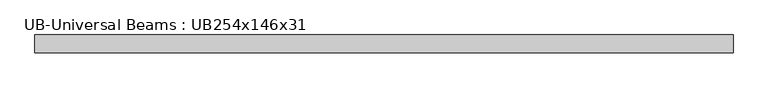
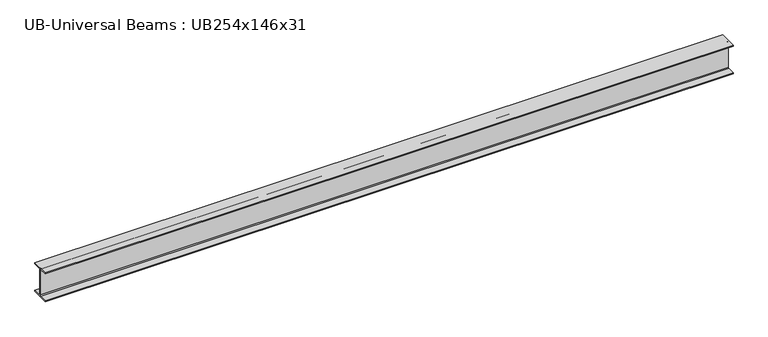
"""IFC4 building model written with IfcOpenShell, lengths in millimetres: beam geometry, UB-Universal Beams : UB254x146x31."""

from ifc_helpers import new_model, si_unit, point, frame, frame_2d, origin, place, context, project, spatial, polyline, circle_curve, trimmed, segment, composite_curve, outline, extrude, source, transform, mapped, element, save


def ub_universal_beams_ub254x146x31_048477c2(model_context):
    return source(origin(), model_context, "Body", "SweptSolid", [
        extrude(outline(composite_curve([segment(polyline([(73.05, -117.1), (73.05, -125.7), (-73.05, -125.7), (-73.05, -117.1), (-10.6, -117.1)]), True, "CONTINUOUS"), segment(trimmed(circle_curve(frame_2d((-10.6, -109.5)), 7.6), [point((-10.6, -117.1))], [point((-3.0, -109.5))], True, "CARTESIAN"), True, "CONTINUOUS"), segment(polyline([(-3.0, -109.5), (-3.0, 109.5)]), True, "CONTINUOUS"), segment(trimmed(circle_curve(frame_2d((-10.6, 109.5)), 7.6), [point((-3.0, 109.5))], [point((-10.6, 117.1))], True, "CARTESIAN"), True, "CONTINUOUS"), segment(polyline([(-10.6, 117.1), (-73.05, 117.1), (-73.05, 125.7), (73.05, 125.7), (73.05, 117.1), (10.6, 117.1)]), True, "CONTINUOUS"), segment(trimmed(circle_curve(frame_2d((10.6, 109.5)), 7.6), [point((10.6, 117.1))], [point((3.0, 109.5))], True, "CARTESIAN"), True, "CONTINUOUS"), segment(polyline([(3.0, 109.5), (3.0, -109.5)]), True, "CONTINUOUS"), segment(trimmed(circle_curve(frame_2d((10.6, -109.5)), 7.6), [point((3.0, -109.5))], [point((10.6, -117.1))], True, "CARTESIAN"), True, "CONTINUOUS"), segment(polyline([(10.6, -117.1), (73.05, -117.1)]), True, "CONTINUOUS")], self_intersect=False)), frame((-2847.0, 0.0, 0.0), z_axis=(1.0, 0.0, 0.0), x_axis=(0.0, 1.0, 0.0)), (0.0, 0.0, 1.0), 5694.0),
    ])


if __name__ == "__main__":
    model = new_model("IFC4")
    model_context = context("Model", 3, world=origin())
    ifc_project = project(units=[si_unit("LENGTHUNIT", "METRE", prefix="MILLI")], contexts=[model_context])
    site = spatial("IfcSite", under=ifc_project)
    building = spatial("IfcBuilding", under=site)
    placement = place(None, origin())
    ub_universal_beams_ub254x146x31_shape = ub_universal_beams_ub254x146x31_048477c2(model_context)
    element("IfcBeam", 1, ObjectType="UB-Universal Beams : UB254x146x31", at=placement, inside=building, context=model_context, shape_type="MappedRepresentation", body=[
        mapped(ub_universal_beams_ub254x146x31_shape, transform((0.0, 0.0, 0.0), x_axis=(1.0, 0.0, 0.0), y_axis=(0.0, 1.0, 0.0), z_axis=(0.0, 0.0, 1.0))),
    ])
    save(model, "model.ifc")

# Revit data of these elements
# Type "UB-Universal Beams : UB254x146x31"
#   Section Name Key = "UB254X146X31"
#   Width = 14.61 cm
#   Web Thickness = 0.6 cm
#   Web Fillet = 0.76 cm
#   Warping Constant = 66000.0 cm⁶
#   Torsional Moment of Inertia = 8.55 cm⁴
#   Section Area = 39.7 cm²
#   Plastic Modulus weak axis = 94.1 cm³
#   Plastic Modulus strong axis = 393.0 cm³
#   Nominal Weight = 31.10 kgf/m
#   Moment of Inertia weak axis = 448.00 cm⁴
#   Moment of Inertia strong axis = 4413.00 cm⁴
#   Height = 25.14 cm
#   Flange Thickness = 0.86 cm
#   Elastic Modulus weak axis = 61.3 cm³
#   Elastic Modulus strong axis = 351.0 cm³
#   Centroid Vertical = 12.57 cm
#   Centroid Horizontal = 7.305 cm
#   Bolt Spacing = 7.0 cm
#   Length [instance default] = 1500 mm
#   Structural Material [instance default] = Metal - Steel 43-275
#   Type Comments = ""
#   Assembly Code = ""
# Element 1 (IfcBeam, "UB-Universal Beams : UB254x146x31")
#   Materials on its faces: "Metal - Steel 43-275"
# Materials
#   "Metal - Steel 43-275": class "Metal", colour RGB 247 247 247, transparency 0, Cost = 0
